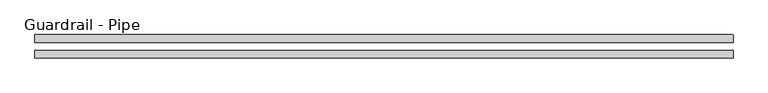
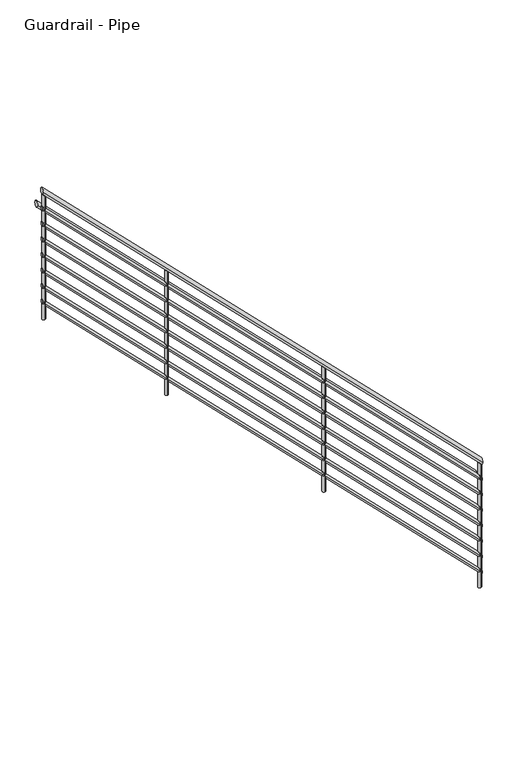
"""IFC4 building model written with IfcOpenShell, lengths in millimetres: railing geometry, Guardrail - Pipe."""

import ifcopenshell
import ifcopenshell.guid

model = None  # the IFC model being written
_history = None  # IfcOwnerHistory: only IFC2X3 demands one
_inside = {}  # id of a spatial element -> (the spatial element, [elements in it])
_under = {}  # id of a project, library or spatial element -> (it, [spatial elements below it])
_declared = {}  # id of a project -> (the project, [libraries it declares])
_typed = {}  # id of a type object -> (the type object, [elements of that type])
_made_of = {}  # id of a material, layer set ... -> (it, [elements and type objects made of it])


def new_model(schema):
    """Start an empty IFC model of exactly this schema.

    Asked for "IFC4X3", IfcOpenShell would pick the latest addendum, in which some entities
    have other attributes; the version numbers below select the first issue.
    IFC2X3 requires an IfcOwnerHistory on every rooted entity: one is made here for all.
    """
    global model, _history
    if schema == "IFC4X3":
        model = ifcopenshell.file(schema_version=(4, 3, 0, 0))
    else:
        model = ifcopenshell.file(schema=schema)
    _inside.clear()
    _under.clear()
    _declared.clear()
    _typed.clear()
    _made_of.clear()
    _history = None
    if model.schema == "IFC2X3":
        org = make("IfcOrganization", Name="unknown")
        user = make(
            "IfcPersonAndOrganization",
            ThePerson=make("IfcPerson", FamilyName="unknown"),
            TheOrganization=org,
        )
        app = make(
            "IfcApplication",
            ApplicationDeveloper=org,
            Version="unknown",
            ApplicationFullName="unknown",
            ApplicationIdentifier="unknown",
        )
        _history = make(
            "IfcOwnerHistory",
            OwningUser=user,
            OwningApplication=app,
            ChangeAction="ADDED",
            CreationDate=0,
        )
    return model


def make(cls, **values):
    """One entity of the class cls with the attributes given. An attribute that is None is left unset."""
    return model.create_entity(
        cls, **{name: value for name, value in values.items() if value is not None}
    )


def rooted(cls, **values):
    """An entity with a GlobalId (a new one), such as an element, a storey or a relation."""
    return make(cls, GlobalId=ifcopenshell.guid.new(), OwnerHistory=_history, **values)


def si_unit(unit_type, name, prefix=None):
    """IfcSIUnit, for example si_unit("LENGTHUNIT", "METRE", prefix="MILLI")."""
    return make("IfcSIUnit", UnitType=unit_type, Prefix=prefix, Name=name)


def assignment(units):
    """IfcUnitAssignment: the units of a project."""
    return None if units is None else make("IfcUnitAssignment", Units=units)


def point(xyz):
    """IfcCartesianPoint."""
    return None if xyz is None else make("IfcCartesianPoint", Coordinates=xyz)


def direction(xyz):
    """IfcDirection."""
    return None if xyz is None else make("IfcDirection", DirectionRatios=xyz)


def frame(location, z_axis=None, x_axis=None):
    """IfcAxis2Placement3D, a coordinate frame: its origin and axes. An axis left out is left unset."""
    return make(
        "IfcAxis2Placement3D",
        Location=point(location),
        Axis=direction(z_axis),
        RefDirection=direction(x_axis),
    )


def origin():
    """The frame at (0, 0, 0) with its axes left unset."""
    return frame((0.0, 0.0, 0.0))


def place(relative_to, where):
    """IfcLocalPlacement: puts the frame where relative to a parent placement (None: the world)."""
    return make(
        "IfcLocalPlacement", PlacementRelTo=relative_to, RelativePlacement=where
    )


def context(
    kind, dimensions, precision=None, world=None, true_north=None, identifier=None
):
    """IfcGeometricRepresentationContext, for example the 3D "Model" context."""
    return make(
        "IfcGeometricRepresentationContext",
        ContextIdentifier=identifier,
        ContextType=kind,
        CoordinateSpaceDimension=dimensions,
        Precision=precision,
        WorldCoordinateSystem=world,
        TrueNorth=true_north,
    )


def project(units=None, contexts=None):
    """IfcProject with its units and contexts."""
    return rooted(
        "IfcProject",
        Name="project",
        RepresentationContexts=contexts,
        UnitsInContext=assignment(units),
    )


def spatial(cls, under=None, at=None, **own):
    """A site, building, storey or space (cls), placed at a placement, below another one or the project."""
    s = rooted(cls, ObjectPlacement=at, **own)
    if under is not None:
        _under.setdefault(under.id(), (under, []))[1].append(s)
    return s


def circle_curve(where, radius):
    """IfcCircle in the frame where."""
    return make("IfcCircle", Position=where, Radius=radius)


def ellipse_curve(where, semi_axis1, semi_axis2):
    """IfcEllipse in the frame where."""
    return make(
        "IfcEllipse", Position=where, SemiAxis1=semi_axis1, SemiAxis2=semi_axis2
    )


def shape(context_of_items, identifier, shape_type, items):
    """IfcShapeRepresentation: the items that make up one representation, for example the "Body"."""
    return make(
        "IfcShapeRepresentation",
        ContextOfItems=context_of_items,
        RepresentationIdentifier=identifier,
        RepresentationType=shape_type,
        Items=items,
    )


def source(mapping_origin, context_of_items, identifier, shape_type, items):
    """IfcRepresentationMap: a shape defined once, which mapped items show again and again."""
    return make(
        "IfcRepresentationMap",
        MappingOrigin=mapping_origin,
        MappedRepresentation=shape(context_of_items, identifier, shape_type, items),
    )


def transform(
    local_origin,
    x_axis=None,
    y_axis=None,
    z_axis=None,
    scale=None,
    scale2=None,
    scale3=None,
    uniform=True,
):
    """IfcCartesianTransformationOperator3D, or its non-uniform kind. x_axis, y_axis, z_axis: its Axis1, 2, 3."""
    if uniform:
        return make(
            "IfcCartesianTransformationOperator3D",
            Axis1=direction(x_axis),
            Axis2=direction(y_axis),
            LocalOrigin=point(local_origin),
            Scale=scale,
            Axis3=direction(z_axis),
        )
    return make(
        "IfcCartesianTransformationOperator3DnonUniform",
        Axis1=direction(x_axis),
        Axis2=direction(y_axis),
        LocalOrigin=point(local_origin),
        Scale=scale,
        Axis3=direction(z_axis),
        Scale2=scale2,
        Scale3=scale3,
    )


def mapped(mapping_source, mapping_target):
    """IfcMappedItem: shows the shape of a source again, moved by a transform."""
    return make(
        "IfcMappedItem", MappingSource=mapping_source, MappingTarget=mapping_target
    )


def made_of(thing, what):
    """Note that an element or type object is made of a material, layer set ...; save() writes the relation."""
    if what is not None:
        _made_of.setdefault(what.id(), (what, []))[1].append(thing)
    return thing


def element(
    cls,
    number,
    at=None,
    inside=None,
    cuts=None,
    type_object=None,
    material=None,
    context=None,
    identifier="Body",
    shape_type=None,
    held_by="IfcProductDefinitionShape",
    body=None,
    shapes=None,
    **own,
):
    """One element of the class cls, such as IfcWall. Its Tag is "e" and its number.

    at: its placement. inside: the storey or other place that contains it. cuts: it is an
    opening in that element (IfcRelVoidsElement). A single representation is given by context,
    identifier, shape_type and body (its items); several are given by shapes. held_by: the class
    of the entity that holds the representations. save() writes the other relations.
    """
    e = rooted(cls, Tag="e%d" % number, ObjectPlacement=at, **own)
    if body is not None:
        shapes = [shape(context, identifier, shape_type, body)]
    if shapes is not None:
        e.Representation = make(held_by, Representations=shapes)
    if inside is not None:
        _inside.setdefault(inside.id(), (inside, []))[1].append(e)
    if cuts is not None:
        rooted(
            "IfcRelVoidsElement", RelatingBuildingElement=cuts, RelatedOpeningElement=e
        )
    if type_object is not None:
        _typed.setdefault(type_object.id(), (type_object, []))[1].append(e)
    return made_of(e, material)


def aggregate(whole, parts):
    """IfcRelAggregates: a whole, such as a stair, and the parts it consists of."""
    return rooted("IfcRelAggregates", RelatingObject=whole, RelatedObjects=parts)


def save(model, path):
    """Write the relations noted so far, then the file.

    IfcRelAggregates (storeys below a building ...), IfcRelContainedInSpatialStructure (elements
    in a storey), IfcRelDefinesByType, IfcRelAssociatesMaterial and IfcRelDeclares: one each for
    every whole, place, type object, material and project.
    """
    for whole, parts in _under.values():
        aggregate(whole, parts)
    for where, things in _inside.values():
        rooted(
            "IfcRelContainedInSpatialStructure",
            RelatedElements=things,
            RelatingStructure=where,
        )
    for kind, things in _typed.values():
        rooted("IfcRelDefinesByType", RelatedObjects=things, RelatingType=kind)
    for what, things in _made_of.values():
        rooted("IfcRelAssociatesMaterial", RelatedObjects=things, RelatingMaterial=what)
    for by, libraries in _declared.values():
        rooted("IfcRelDeclares", RelatingContext=by, RelatedDefinitions=libraries)
    model.write(path)


def plane_surface(at):
    """IfcPlane: the flat surface through the origin of the frame at, square to its z axis."""
    return make("IfcPlane", Position=at)


def cylinder_surface(at, radius):
    """IfcCylindricalSurface: all points at the distance radius from the z axis of the frame at."""
    return make("IfcCylindricalSurface", Position=at, Radius=radius)


def advanced_brep(points, edges, surfaces, faces):
    """IfcAdvancedBrep: a solid bounded by faces that lie on surfaces and meet in shared edges.

    An edge is (start, end): straight between two places in points (the first is 0);
    or (start, end, curve); or (start, end, curve, False) where it runs against its curve.
    A face is (place in surfaces, loops), or (place, loops, False) where it looks against
    its surface's normal. A loop lists edges by number (the first is 1), with a minus sign
    where the edge is run from its end to its start. The first loop is the outer one.
    """
    corners = [point(p) for p in points]
    vertices = [make("IfcVertexPoint", VertexGeometry=c) for c in corners]
    made = []
    for start, end, *more in edges:
        made.append(
            make(
                "IfcEdgeCurve",
                EdgeStart=vertices[start],
                EdgeEnd=vertices[end],
                EdgeGeometry=more[0] if more else make("IfcPolyline", Points=[corners[start], corners[end]]),
                SameSense=more[1] if len(more) > 1 else True,
            )
        )
    hull = []
    for where, loops, *sense in faces:
        bounds = []
        for j, loop in enumerate(loops):
            ring = [make("IfcOrientedEdge", EdgeElement=made[abs(k) - 1], Orientation=k > 0) for k in loop]
            bounds.append(
                make(
                    "IfcFaceOuterBound" if j == 0 else "IfcFaceBound",
                    Bound=make("IfcEdgeLoop", EdgeList=ring),
                    Orientation=True,
                )
            )
        hull.append(make("IfcAdvancedFace", Bounds=bounds, FaceSurface=surfaces[where], SameSense=sense[0] if sense else True))
    return make("IfcAdvancedBrep", Outer=make("IfcClosedShell", CfsFaces=hull))


def guardrail_pipe_3270e9bd(model_context):
    return source(origin(), model_context, "Body", "AdvancedBrep", [
        advanced_brep(
        [(-7243.3085296, -4922.0836772, 1268.4592316), (-7243.3085296, -4960.1836772, 1268.4592316), (-10645.1029016, -4922.0836772, 4670.2536037), (-10645.1029016, -4960.1836772, 4670.2536037)],
        [
            (0, 1, ellipse_curve(frame((-7243.3085296, -4941.1336772, 1268.4592316), z_axis=(1.0, 0.0, 0.0), x_axis=(0.0, 0.0, -1.0)), 26.9407684, 19.05)),
            (1, 0, ellipse_curve(frame((-7243.3085296, -4941.1336772, 1268.4592316), z_axis=(1.0, 0.0, 0.0), x_axis=(0.0, 0.0, -1.0)), 26.9407684, 19.05)),
            (2, 3, ellipse_curve(frame((-10645.1029016, -4941.1336772, 4670.2536037), z_axis=(-1.0, 0.0, 0.0), x_axis=(0.0, 0.0, -1.0)), 26.9407684, 19.05)),
            (3, 2, ellipse_curve(frame((-10645.1029016, -4941.1336772, 4670.2536037), z_axis=(-1.0, 0.0, 0.0), x_axis=(0.0, 0.0, -1.0)), 26.9407684, 19.05)),
            (0, 2),
            (3, 1),
        ],
        [
            plane_surface(frame((-7243.3085296, -4941.1336772, 1295.4), z_axis=(1.0, 0.0, 0.0), x_axis=(0.0, -1.0, 0.0))),
            plane_surface(frame((-10645.1029016, -4941.1336772, 4697.194372), z_axis=(-1.0, 0.0, 0.0), x_axis=(0.0, -1.0, 0.0))),
            cylinder_surface(frame((-7256.7789137, -4941.1336772, 1281.9296158), z_axis=(0.7071067811865476, 0.0, -0.7071067811865476), x_axis=(0.0, -1.0, 0.0)), 19.05),
        ],
        [
            (0, [[1, 2]]),
            (1, [[3, 4]]),
            (2, [[-1, 5, -4, 6]]),
            (2, [[-2, -6, -3, -5]]),
        ],
    ),
        advanced_brep(
        [(-7243.3085296, -4928.4336772, 1125.0394878), (-7243.3085296, -4953.8336772, 1125.0394878), (-10645.1029016, -4928.4336772, 4526.8338598), (-10645.1029016, -4953.8336772, 4526.8338598)],
        [
            (0, 1, ellipse_curve(frame((-7243.3085296, -4941.1336772, 1125.0394878), z_axis=(1.0, 0.0, 0.0), x_axis=(0.0, 0.0, -1.0)), 17.9605122, 12.7)),
            (1, 0, ellipse_curve(frame((-7243.3085296, -4941.1336772, 1125.0394878), z_axis=(1.0, 0.0, 0.0), x_axis=(0.0, 0.0, -1.0)), 17.9605122, 12.7)),
            (2, 3, ellipse_curve(frame((-10645.1029016, -4941.1336772, 4526.8338598), z_axis=(-1.0, 0.0, 0.0), x_axis=(0.0, 0.0, -1.0)), 17.9605122, 12.7)),
            (3, 2, ellipse_curve(frame((-10645.1029016, -4941.1336772, 4526.8338598), z_axis=(-1.0, 0.0, 0.0), x_axis=(0.0, 0.0, -1.0)), 17.9605122, 12.7)),
            (0, 2),
            (3, 1),
        ],
        [
            plane_surface(frame((-7243.3085296, -4941.1336772, 1143.0), z_axis=(1.0, 0.0, 0.0), x_axis=(0.0, -1.0, 0.0))),
            plane_surface(frame((-10645.1029016, -4941.1336772, 4544.794372), z_axis=(-1.0, 0.0, 0.0), x_axis=(0.0, -1.0, 0.0))),
            cylinder_surface(frame((-7252.2887857, -4941.1336772, 1134.0197439), z_axis=(0.7071067811865476, 0.0, -0.7071067811865476), x_axis=(0.0, -1.0, 0.0)), 12.7),
        ],
        [
            (0, [[1, 2]]),
            (1, [[3, 4]]),
            (2, [[-1, 5, -4, 6]]),
            (2, [[-2, -6, -3, -5]]),
        ],
    ),
        advanced_brep(
        [(-7243.3085296, -4845.8836772, 1116.0592316), (-7243.3085296, -4883.9836772, 1116.0592316), (-10645.1029016, -4845.8836772, 4517.8536037), (-10645.1029016, -4883.9836772, 4517.8536037)],
        [
            (0, 1, ellipse_curve(frame((-7243.3085296, -4864.9336772, 1116.0592316), z_axis=(1.0, 0.0, 0.0), x_axis=(0.0, 0.0, -1.0)), 26.9407684, 19.05)),
            (1, 0, ellipse_curve(frame((-7243.3085296, -4864.9336772, 1116.0592316), z_axis=(1.0, 0.0, 0.0), x_axis=(0.0, 0.0, -1.0)), 26.9407684, 19.05)),
            (2, 3, ellipse_curve(frame((-10645.1029016, -4864.9336772, 4517.8536037), z_axis=(-1.0, 0.0, 0.0), x_axis=(0.0, 0.0, -1.0)), 26.9407684, 19.05)),
            (3, 2, ellipse_curve(frame((-10645.1029016, -4864.9336772, 4517.8536037), z_axis=(-1.0, 0.0, 0.0), x_axis=(0.0, 0.0, -1.0)), 26.9407684, 19.05)),
            (0, 2),
            (3, 1),
        ],
        [
            plane_surface(frame((-7243.3085296, -4864.9336772, 1143.0), z_axis=(1.0, 0.0, 0.0), x_axis=(0.0, -1.0, 0.0))),
            plane_surface(frame((-10645.1029016, -4864.9336772, 4544.794372), z_axis=(-1.0, 0.0, 0.0), x_axis=(0.0, -1.0, 0.0))),
            cylinder_surface(frame((-7256.7789137, -4864.9336772, 1129.5296158), z_axis=(0.7071067811865476, 0.0, -0.7071067811865476), x_axis=(0.0, -1.0, 0.0)), 19.05),
        ],
        [
            (0, [[1, 2]]),
            (1, [[3, 4]]),
            (2, [[-1, 5, -4, 6]]),
            (2, [[-2, -6, -3, -5]]),
        ],
    ),
        advanced_brep(
        [(-7243.3085296, -4928.4336772, 998.0394878), (-7243.3085296, -4953.8336772, 998.0394878), (-10645.1029016, -4928.4336772, 4399.8338598), (-10645.1029016, -4953.8336772, 4399.8338598)],
        [
            (0, 1, ellipse_curve(frame((-7243.3085296, -4941.1336772, 998.0394878), z_axis=(1.0, 0.0, 0.0), x_axis=(0.0, 0.0, -1.0)), 17.9605122, 12.7)),
            (1, 0, ellipse_curve(frame((-7243.3085296, -4941.1336772, 998.0394878), z_axis=(1.0, 0.0, 0.0), x_axis=(0.0, 0.0, -1.0)), 17.9605122, 12.7)),
            (2, 3, ellipse_curve(frame((-10645.1029016, -4941.1336772, 4399.8338598), z_axis=(-1.0, 0.0, 0.0), x_axis=(0.0, 0.0, -1.0)), 17.9605122, 12.7)),
            (3, 2, ellipse_curve(frame((-10645.1029016, -4941.1336772, 4399.8338598), z_axis=(-1.0, 0.0, 0.0), x_axis=(0.0, 0.0, -1.0)), 17.9605122, 12.7)),
            (0, 2),
            (3, 1),
        ],
        [
            plane_surface(frame((-7243.3085296, -4941.1336772, 1016.0), z_axis=(1.0, 0.0, 0.0), x_axis=(0.0, -1.0, 0.0))),
            plane_surface(frame((-10645.1029016, -4941.1336772, 4417.794372), z_axis=(-1.0, 0.0, 0.0), x_axis=(0.0, -1.0, 0.0))),
            cylinder_surface(frame((-7252.2887857, -4941.1336772, 1007.0197439), z_axis=(0.7071067811865476, 0.0, -0.7071067811865476), x_axis=(0.0, -1.0, 0.0)), 12.7),
        ],
        [
            (0, [[1, 2]]),
            (1, [[3, 4]]),
            (2, [[-1, 5, -4, 6]]),
            (2, [[-2, -6, -3, -5]]),
        ],
    ),
        advanced_brep(
        [(-7243.3085296, -4928.4336772, 871.0394878), (-7243.3085296, -4953.8336772, 871.0394878), (-10645.1029016, -4928.4336772, 4272.8338598), (-10645.1029016, -4953.8336772, 4272.8338598)],
        [
            (0, 1, ellipse_curve(frame((-7243.3085296, -4941.1336772, 871.0394878), z_axis=(1.0, 0.0, 0.0), x_axis=(0.0, 0.0, -1.0)), 17.9605122, 12.7)),
            (1, 0, ellipse_curve(frame((-7243.3085296, -4941.1336772, 871.0394878), z_axis=(1.0, 0.0, 0.0), x_axis=(0.0, 0.0, -1.0)), 17.9605122, 12.7)),
            (2, 3, ellipse_curve(frame((-10645.1029016, -4941.1336772, 4272.8338598), z_axis=(-1.0, 0.0, 0.0), x_axis=(0.0, 0.0, -1.0)), 17.9605122, 12.7)),
            (3, 2, ellipse_curve(frame((-10645.1029016, -4941.1336772, 4272.8338598), z_axis=(-1.0, 0.0, 0.0), x_axis=(0.0, 0.0, -1.0)), 17.9605122, 12.7)),
            (0, 2),
            (3, 1),
        ],
        [
            plane_surface(frame((-7243.3085296, -4941.1336772, 889.0), z_axis=(1.0, 0.0, 0.0), x_axis=(0.0, -1.0, 0.0))),
            plane_surface(frame((-10645.1029016, -4941.1336772, 4290.794372), z_axis=(-1.0, 0.0, 0.0), x_axis=(0.0, -1.0, 0.0))),
            cylinder_surface(frame((-7252.2887857, -4941.1336772, 880.0197439), z_axis=(0.7071067811865476, 0.0, -0.7071067811865476), x_axis=(0.0, -1.0, 0.0)), 12.7),
        ],
        [
            (0, [[1, 2]]),
            (1, [[3, 4]]),
            (2, [[-1, 5, -4, 6]]),
            (2, [[-2, -6, -3, -5]]),
        ],
    ),
        advanced_brep(
        [(-7243.3085296, -4928.4336772, 744.0394878), (-7243.3085296, -4953.8336772, 744.0394878), (-10645.1029016, -4928.4336772, 4145.8338598), (-10645.1029016, -4953.8336772, 4145.8338598)],
        [
            (0, 1, ellipse_curve(frame((-7243.3085296, -4941.1336772, 744.0394878), z_axis=(1.0, 0.0, 0.0), x_axis=(0.0, 0.0, -1.0)), 17.9605122, 12.7)),
            (1, 0, ellipse_curve(frame((-7243.3085296, -4941.1336772, 744.0394878), z_axis=(1.0, 0.0, 0.0), x_axis=(0.0, 0.0, -1.0)), 17.9605122, 12.7)),
            (2, 3, ellipse_curve(frame((-10645.1029016, -4941.1336772, 4145.8338598), z_axis=(-1.0, 0.0, 0.0), x_axis=(0.0, 0.0, -1.0)), 17.9605122, 12.7)),
            (3, 2, ellipse_curve(frame((-10645.1029016, -4941.1336772, 4145.8338598), z_axis=(-1.0, 0.0, 0.0), x_axis=(0.0, 0.0, -1.0)), 17.9605122, 12.7)),
            (0, 2),
            (3, 1),
        ],
        [
            plane_surface(frame((-7243.3085296, -4941.1336772, 762.0), z_axis=(1.0, 0.0, 0.0), x_axis=(0.0, -1.0, 0.0))),
            plane_surface(frame((-10645.1029016, -4941.1336772, 4163.794372), z_axis=(-1.0, 0.0, 0.0), x_axis=(0.0, -1.0, 0.0))),
            cylinder_surface(frame((-7252.2887857, -4941.1336772, 753.0197439), z_axis=(0.7071067811865476, 0.0, -0.7071067811865476), x_axis=(0.0, -1.0, 0.0)), 12.7),
        ],
        [
            (0, [[1, 2]]),
            (1, [[3, 4]]),
            (2, [[-1, 5, -4, 6]]),
            (2, [[-2, -6, -3, -5]]),
        ],
    ),
        advanced_brep(
        [(-7243.3085296, -4928.4336772, 617.0394878), (-7243.3085296, -4953.8336772, 617.0394878), (-10645.1029016, -4928.4336772, 4018.8338598), (-10645.1029016, -4953.8336772, 4018.8338598)],
        [
            (0, 1, ellipse_curve(frame((-7243.3085296, -4941.1336772, 617.0394878), z_axis=(1.0, 0.0, 0.0), x_axis=(0.0, 0.0, -1.0)), 17.9605122, 12.7)),
            (1, 0, ellipse_curve(frame((-7243.3085296, -4941.1336772, 617.0394878), z_axis=(1.0, 0.0, 0.0), x_axis=(0.0, 0.0, -1.0)), 17.9605122, 12.7)),
            (2, 3, ellipse_curve(frame((-10645.1029016, -4941.1336772, 4018.8338598), z_axis=(-1.0, 0.0, 0.0), x_axis=(0.0, 0.0, -1.0)), 17.9605122, 12.7)),
            (3, 2, ellipse_curve(frame((-10645.1029016, -4941.1336772, 4018.8338598), z_axis=(-1.0, 0.0, 0.0), x_axis=(0.0, 0.0, -1.0)), 17.9605122, 12.7)),
            (0, 2),
            (3, 1),
        ],
        [
            plane_surface(frame((-7243.3085296, -4941.1336772, 635.0), z_axis=(1.0, 0.0, 0.0), x_axis=(0.0, -1.0, 0.0))),
            plane_surface(frame((-10645.1029016, -4941.1336772, 4036.794372), z_axis=(-1.0, 0.0, 0.0), x_axis=(0.0, -1.0, 0.0))),
            cylinder_surface(frame((-7252.2887857, -4941.1336772, 626.0197439), z_axis=(0.7071067811865476, 0.0, -0.7071067811865476), x_axis=(0.0, -1.0, 0.0)), 12.7),
        ],
        [
            (0, [[1, 2]]),
            (1, [[3, 4]]),
            (2, [[-1, 5, -4, 6]]),
            (2, [[-2, -6, -3, -5]]),
        ],
    ),
        advanced_brep(
        [(-7243.3085296, -4928.4336772, 490.0394878), (-7243.3085296, -4953.8336772, 490.0394878), (-10645.1029016, -4928.4336772, 3891.8338598), (-10645.1029016, -4953.8336772, 3891.8338598)],
        [
            (0, 1, ellipse_curve(frame((-7243.3085296, -4941.1336772, 490.0394878), z_axis=(1.0, 0.0, 0.0), x_axis=(0.0, 0.0, -1.0)), 17.9605122, 12.7)),
            (1, 0, ellipse_curve(frame((-7243.3085296, -4941.1336772, 490.0394878), z_axis=(1.0, 0.0, 0.0), x_axis=(0.0, 0.0, -1.0)), 17.9605122, 12.7)),
            (2, 3, ellipse_curve(frame((-10645.1029016, -4941.1336772, 3891.8338598), z_axis=(-1.0, 0.0, 0.0), x_axis=(0.0, 0.0, -1.0)), 17.9605122, 12.7)),
            (3, 2, ellipse_curve(frame((-10645.1029016, -4941.1336772, 3891.8338598), z_axis=(-1.0, 0.0, 0.0), x_axis=(0.0, 0.0, -1.0)), 17.9605122, 12.7)),
            (0, 2),
            (3, 1),
        ],
        [
            plane_surface(frame((-7243.3085296, -4941.1336772, 508.0), z_axis=(1.0, 0.0, 0.0), x_axis=(0.0, -1.0, 0.0))),
            plane_surface(frame((-10645.1029016, -4941.1336772, 3909.794372), z_axis=(-1.0, 0.0, 0.0), x_axis=(0.0, -1.0, 0.0))),
            cylinder_surface(frame((-7252.2887857, -4941.1336772, 499.0197439), z_axis=(0.7071067811865476, 0.0, -0.7071067811865476), x_axis=(0.0, -1.0, 0.0)), 12.7),
        ],
        [
            (0, [[1, 2]]),
            (1, [[3, 4]]),
            (2, [[-1, 5, -4, 6]]),
            (2, [[-2, -6, -3, -5]]),
        ],
    ),
        advanced_brep(
        [(-7243.3085296, -4928.4336772, 363.0394878), (-7243.3085296, -4953.8336772, 363.0394878), (-10645.1029016, -4928.4336772, 3764.8338598), (-10645.1029016, -4953.8336772, 3764.8338598)],
        [
            (0, 1, ellipse_curve(frame((-7243.3085296, -4941.1336772, 363.0394878), z_axis=(1.0, 0.0, 0.0), x_axis=(0.0, 0.0, -1.0)), 17.9605122, 12.7)),
            (1, 0, ellipse_curve(frame((-7243.3085296, -4941.1336772, 363.0394878), z_axis=(1.0, 0.0, 0.0), x_axis=(0.0, 0.0, -1.0)), 17.9605122, 12.7)),
            (2, 3, ellipse_curve(frame((-10645.1029016, -4941.1336772, 3764.8338598), z_axis=(-1.0, 0.0, 0.0), x_axis=(0.0, 0.0, -1.0)), 17.9605122, 12.7)),
            (3, 2, ellipse_curve(frame((-10645.1029016, -4941.1336772, 3764.8338598), z_axis=(-1.0, 0.0, 0.0), x_axis=(0.0, 0.0, -1.0)), 17.9605122, 12.7)),
            (0, 2),
            (3, 1),
        ],
        [
            plane_surface(frame((-7243.3085296, -4941.1336772, 381.0), z_axis=(1.0, 0.0, 0.0), x_axis=(0.0, -1.0, 0.0))),
            plane_surface(frame((-10645.1029016, -4941.1336772, 3782.794372), z_axis=(-1.0, 0.0, 0.0), x_axis=(0.0, -1.0, 0.0))),
            cylinder_surface(frame((-7252.2887857, -4941.1336772, 372.0197439), z_axis=(0.7071067811865476, 0.0, -0.7071067811865476), x_axis=(0.0, -1.0, 0.0)), 12.7),
        ],
        [
            (0, [[1, 2]]),
            (1, [[3, 4]]),
            (2, [[-1, 5, -4, 6]]),
            (2, [[-2, -6, -3, -5]]),
        ],
    ),
        advanced_brep(
        [(-9681.7085296, -4953.8336772, 3679.9184633), (-9681.7085296, -4928.4336772, 3679.9184633), (-9681.7085296, -4928.4336772, 2667.0), (-9681.7085296, -4953.8336772, 2667.0)],
        [
            (0, 1, ellipse_curve(frame((-9681.7085296, -4941.1336772, 3679.9184633), z_axis=(-0.7071067811865471, 0.0, -0.7071067811865479), x_axis=(-0.7071067811865479, 0.0, 0.7071067811865471)), 17.9605122, 12.7)),
            (1, 2),
            (2, 3, circle_curve(frame((-9681.7085296, -4941.1336772, 2667.0), z_axis=(0.0, 0.0, 1.0), x_axis=(0.0, 1.0, 0.0)), 12.7)),
            (3, 0),
            (3, 2, circle_curve(frame((-9681.7085296, -4941.1336772, 2667.0), z_axis=(0.0, 0.0, 1.0), x_axis=(0.0, 1.0, 0.0)), 12.7)),
            (1, 0, ellipse_curve(frame((-9681.7085296, -4941.1336772, 3679.9184633), z_axis=(-0.7071067811865471, 0.0, -0.7071067811865479), x_axis=(-0.7071067811865479, 0.0, 0.7071067811865471)), 17.9605122, 12.7)),
        ],
        [
            cylinder_surface(frame((-9681.7085296, -4941.1336772, 2438.4), z_axis=(0.0, 0.0, 1.0), x_axis=(0.0, 1.0, 0.0)), 12.7),
            plane_surface(frame((-9707.1085296, -4915.7336772, 3705.3184633), z_axis=(0.7071067811865471, 0.0, 0.7071067811865479), x_axis=(0.0, -1.0, 0.0))),
            plane_surface(frame((-9656.3085296, -4915.7336772, 2667.0), z_axis=(0.0, 0.0, -1.0), x_axis=(0.0, -1.0, 0.0))),
        ],
        [
            (0, [[1, 2, 3, 4]]),
            (0, [[5, -2, 6, -4]]),
            (1, [[-6, -1]]),
            (2, [[-5, -3]]),
        ],
    ),
        advanced_brep(
        [(-8462.5085296, -4953.8336772, 2460.7184633), (-8462.5085296, -4928.4336772, 2460.7184633), (-8462.5085296, -4928.4336772, 1447.8), (-8462.5085296, -4953.8336772, 1447.8)],
        [
            (0, 1, ellipse_curve(frame((-8462.5085296, -4941.1336772, 2460.7184633), z_axis=(-0.7071067811865471, 0.0, -0.7071067811865479), x_axis=(-0.7071067811865479, 0.0, 0.7071067811865471)), 17.9605122, 12.7)),
            (1, 2),
            (2, 3, circle_curve(frame((-8462.5085296, -4941.1336772, 1447.8), z_axis=(0.0, 0.0, 1.0), x_axis=(0.0, 1.0, 0.0)), 12.7)),
            (3, 0),
            (3, 2, circle_curve(frame((-8462.5085296, -4941.1336772, 1447.8), z_axis=(0.0, 0.0, 1.0), x_axis=(0.0, 1.0, 0.0)), 12.7)),
            (1, 0, ellipse_curve(frame((-8462.5085296, -4941.1336772, 2460.7184633), z_axis=(-0.7071067811865471, 0.0, -0.7071067811865479), x_axis=(-0.7071067811865479, 0.0, 0.7071067811865471)), 17.9605122, 12.7)),
        ],
        [
            cylinder_surface(frame((-8462.5085296, -4941.1336772, 1219.2), z_axis=(0.0, 0.0, 1.0), x_axis=(0.0, 1.0, 0.0)), 12.7),
            plane_surface(frame((-8487.9085296, -4915.7336772, 2486.1184633), z_axis=(0.7071067811865471, 0.0, 0.7071067811865479), x_axis=(0.0, -1.0, 0.0))),
            plane_surface(frame((-8437.1085296, -4915.7336772, 1447.8), z_axis=(0.0, 0.0, -1.0), x_axis=(0.0, -1.0, 0.0))),
        ],
        [
            (0, [[1, 2, 3, 4]]),
            (0, [[5, -2, 6, -4]]),
            (1, [[-6, -1]]),
            (2, [[-5, -3]]),
        ],
    ),
        advanced_brep(
        [(-10632.4029016, -4953.8336772, 4630.6128353), (-10632.4029016, -4928.4336772, 4630.6128353), (-10632.4029016, -4928.4336772, 3617.694372), (-10632.4029016, -4953.8336772, 3617.694372)],
        [
            (0, 1, ellipse_curve(frame((-10632.4029016, -4941.1336772, 4630.6128353), z_axis=(-0.7071067811865471, 0.0, -0.7071067811865479), x_axis=(-0.7071067811865479, 0.0, 0.7071067811865471)), 17.9605122, 12.7)),
            (1, 2),
            (2, 3, circle_curve(frame((-10632.4029016, -4941.1336772, 3617.694372), z_axis=(0.0, 0.0, 1.0), x_axis=(0.0, 1.0, 0.0)), 12.7)),
            (3, 0),
            (3, 2, circle_curve(frame((-10632.4029016, -4941.1336772, 3617.694372), z_axis=(0.0, 0.0, 1.0), x_axis=(0.0, 1.0, 0.0)), 12.7)),
            (1, 0, ellipse_curve(frame((-10632.4029016, -4941.1336772, 4630.6128353), z_axis=(-0.7071067811865471, 0.0, -0.7071067811865479), x_axis=(-0.7071067811865479, 0.0, 0.7071067811865471)), 17.9605122, 12.7)),
        ],
        [
            cylinder_surface(frame((-10632.4029016, -4941.1336772, 3389.094372), z_axis=(0.0, 0.0, 1.0), x_axis=(0.0, 1.0, 0.0)), 12.7),
            plane_surface(frame((-10657.8029016, -4915.7336772, 4656.0128353), z_axis=(0.7071067811865471, 0.0, 0.7071067811865479), x_axis=(0.0, -1.0, 0.0))),
            plane_surface(frame((-10607.0029016, -4915.7336772, 3617.694372), z_axis=(0.0, 0.0, -1.0), x_axis=(0.0, -1.0, 0.0))),
        ],
        [
            (0, [[1, 2, 3, 4]]),
            (0, [[5, -2, 6, -4]]),
            (1, [[-6, -1]]),
            (2, [[-5, -3]]),
        ],
    ),
        advanced_brep(
        [(-7256.0085296, -4953.8336772, 1254.2184633), (-7256.0085296, -4928.4336772, 1254.2184633), (-7256.0085296, -4928.4336772, 241.3), (-7256.0085296, -4953.8336772, 241.3)],
        [
            (0, 1, ellipse_curve(frame((-7256.0085296, -4941.1336772, 1254.2184633), z_axis=(-0.7071067811865471, 0.0, -0.7071067811865479), x_axis=(-0.7071067811865479, 0.0, 0.7071067811865471)), 17.9605122, 12.7)),
            (1, 2),
            (2, 3, circle_curve(frame((-7256.0085296, -4941.1336772, 241.3), z_axis=(0.0, 0.0, 1.0), x_axis=(0.0, 1.0, 0.0)), 12.7)),
            (3, 0),
            (3, 2, circle_curve(frame((-7256.0085296, -4941.1336772, 241.3), z_axis=(0.0, 0.0, 1.0), x_axis=(0.0, 1.0, 0.0)), 12.7)),
            (1, 0, ellipse_curve(frame((-7256.0085296, -4941.1336772, 1254.2184633), z_axis=(-0.7071067811865471, 0.0, -0.7071067811865479), x_axis=(-0.7071067811865479, 0.0, 0.7071067811865471)), 17.9605122, 12.7)),
        ],
        [
            cylinder_surface(frame((-7256.0085296, -4941.1336772, 12.7), z_axis=(0.0, 0.0, 1.0), x_axis=(0.0, 1.0, 0.0)), 12.7),
            plane_surface(frame((-7281.4085296, -4915.7336772, 1279.6184633), z_axis=(0.7071067811865471, 0.0, 0.7071067811865479), x_axis=(0.0, -1.0, 0.0))),
            plane_surface(frame((-7230.6085296, -4915.7336772, 241.3), z_axis=(0.0, 0.0, -1.0), x_axis=(0.0, -1.0, 0.0))),
        ],
        [
            (0, [[1, 2, 3, 4]]),
            (0, [[5, -2, 6, -4]]),
            (1, [[-6, -1]]),
            (2, [[-5, -3]]),
        ],
    ),
    ])


if __name__ == "__main__":
    model = new_model("IFC4")
    model_context = context("Model", 3, world=origin())
    ifc_project = project(units=[si_unit("LENGTHUNIT", "METRE", prefix="MILLI")], contexts=[model_context])
    site = spatial("IfcSite", under=ifc_project)
    building = spatial("IfcBuilding", under=site)
    placement = place(None, origin())
    guardrail_pipe_shape = guardrail_pipe_3270e9bd(model_context)
    element("IfcRailing", 1, ObjectType="Guardrail - Pipe", at=placement, inside=building, context=model_context, shape_type="MappedRepresentation", body=[
        mapped(guardrail_pipe_shape, transform((0.0, 0.0, 0.0), x_axis=(1.0, 0.0, 0.0), y_axis=(0.0, 1.0, 0.0), z_axis=(0.0, 0.0, 1.0))),
    ])
    save(model, "model.ifc")

# Revit data of these elements
# Element 1 (IfcRailing, "Guardrail - Pipe")
#   Materials on its faces: "Plastic - Vinyl Cove Base"
# Materials
#   "Plastic - Vinyl Cove Base": class "Plastic", colour RGB 5 5 5, transparency 0, Cost = 0
